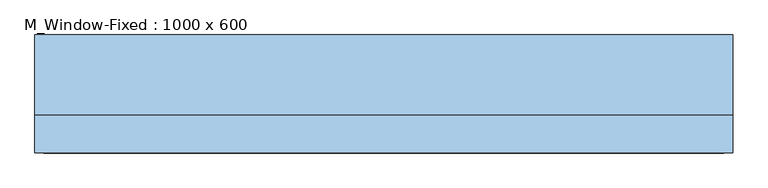
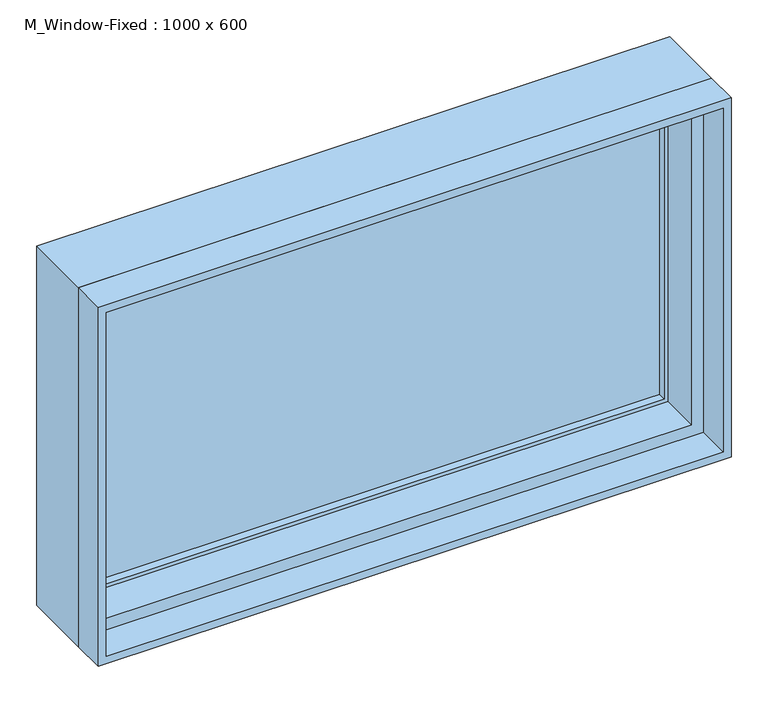
"""IFC4 building model written with IfcOpenShell, lengths in millimetres: window geometry, M_Window-Fixed : 1000 x 600."""

from ifc_helpers import new_model, si_unit, frame, origin, place, context, project, spatial, polyline, outline, extrude, faceted_brep, source, transform, mapped, element, save


def m_window_fixed_1000_x_600_225995cc(model_context):
    return source(origin(), model_context, "Body", "SolidModel", [
        faceted_brep([(500.0, -20.25, 1500.0), (500.0, 94.05, 1500.0), (-500.0, 94.05, 1500.0), (-500.0, -20.25, 1500.0), (-500.0, 94.05, 900.0), (-500.0, -20.25, 900.0), (500.0, 94.05, 900.0), (500.0, -20.25, 900.0), (468.25, -20.25, 1468.25), (468.25, -20.25, 931.75), (-468.25, -20.25, 931.75), (-468.25, -20.25, 1468.25), (-487.3, 94.05, 1487.3), (-487.3, 94.05, 912.7), (487.3, 94.05, 912.7), (487.3, 94.05, 1487.3), (468.25, 43.25, 1468.25), (-468.25, 43.25, 1468.25), (487.3, 43.25, 1487.3), (-487.3, 43.25, 1487.3), (-468.25, 43.25, 931.75), (-487.3, 43.25, 912.7), (468.25, 43.25, 931.75), (487.3, 43.25, 912.7)], [[[0, 1, 2, 3]], [[3, 2, 4, 5]], [[5, 4, 6, 7]], [[3, 5, 7, 0], [8, 9, 10, 11]], [[7, 6, 1, 0]], [[1, 6, 4, 2], [12, 13, 14, 15]], [[16, 8, 11, 17]], [[15, 18, 19, 12]], [[17, 11, 10, 20]], [[12, 19, 21, 13]], [[20, 10, 9, 22]], [[13, 21, 23, 14]], [[22, 9, 8, 16]], [[18, 23, 21, 19], [17, 20, 22, 16]], [[14, 23, 18, 15]]]),
        extrude(outline(polyline([(1500.0, -500.0), (900.0, -500.0), (900.0, 500.0), (1500.0, 500.0), (1500.0, -500.0)]), holes=[polyline([(1487.3, 487.3), (912.7, 487.3), (912.7, -487.3), (1487.3, -487.3), (1487.3, 487.3)])]), frame((0.0, -75.0, 0.0), z_axis=(0.0, 1.0, 0.0), x_axis=(0.0, 0.0, 1.0)), (0.0, 0.0, 1.0), 54.75),
        extrude(outline(polyline([(912.7, 487.3), (1487.3, 487.3), (1487.3, -487.3), (912.7, -487.3), (912.7, 487.3)]), holes=[polyline([(938.1, -461.9), (1461.9, -461.9), (1461.9, 461.9), (938.1, 461.9), (938.1, -461.9)])]), frame((0.0, 43.25, 0.0), z_axis=(0.0, 1.0, 0.0), x_axis=(0.0, 0.0, 1.0)), (0.0, 0.0, 1.0), 44.45),
        extrude(outline(polyline([(461.9, 75.0), (461.9, 68.65), (-461.9, 68.65), (-461.9, 75.0), (461.9, 75.0)])), frame((0.0, 0.0, 938.1), z_axis=(0.0, 0.0, 1.0), x_axis=(1.0, 0.0, 0.0)), (0.0, 0.0, 1.0), 523.8),
        extrude(outline(polyline([(-461.9, 55.95), (-461.9, 62.3), (461.9, 62.3), (461.9, 55.95), (-461.9, 55.95)])), frame((0.0, 0.0, 938.1), z_axis=(0.0, 0.0, 1.0), x_axis=(1.0, 0.0, 0.0)), (0.0, 0.0, 1.0), 523.8),
    ])


if __name__ == "__main__":
    model = new_model("IFC4")
    model_context = context("Model", 3, world=origin())
    ifc_project = project(units=[si_unit("LENGTHUNIT", "METRE", prefix="MILLI")], contexts=[model_context])
    site = spatial("IfcSite", under=ifc_project)
    building = spatial("IfcBuilding", under=site)
    placement = place(None, origin())
    m_window_fixed_1000_x_600_shape = m_window_fixed_1000_x_600_225995cc(model_context)
    element("IfcWindow", 1, ObjectType="M_Window-Fixed : 1000 x 600", at=placement, inside=building, context=model_context, shape_type="MappedRepresentation", body=[
        mapped(m_window_fixed_1000_x_600_shape, transform((0.0, 0.0, 0.0), x_axis=(1.0, 0.0, 0.0), y_axis=(0.0, 1.0, 0.0), z_axis=(0.0, 0.0, 1.0))),
    ])
    save(model, "model.ifc")

# Revit data of these elements
# Type "M_Window-Fixed : 1000 x 600"
#   Type Mark = "42"
#   Fire Rating = "0.5h"
#   Assembly Code = "B2020100"
#   Analytic Construction = "Double glazing - domestic"
#   Window Inset [instance default] = 0 mm
#   Wall Thickness [instance default] = 150 mm
#   Visual Light Transmittance = 0.81
#   Thermal Resistance (R) = 0.319569 (m²·K)/W
#   Solar Heat Gain Coefficient = 0.76
#   Rough Width = 1015 mm
#   Rough Height = 615 mm
#   Interior Wall Closure [instance default] = 54.75 mm
#   Height = 600 mm
#   Heat Transfer Coefficient (U) = 3.12929 W/(m²·K)
#   Frame Extension [instance default] = 6.35 mm
#   Exterior Wall Closure [instance default] = 31.75 mm
#   Extension Jamb [instance default] = 54.75 mm
#   Default Sill Height = 900 mm
#   Width = 1000 mm
#   Muntin Visibility = yes
#   Interior Trim Visibility [instance default] = yes
#   Exterior Trim Visibility [instance default] = yes
#   Extension Jamb Visibility [instance default] = yes
#   Muntin Pattern = M_Muntin Pattern_2x2 : M_Muntin Pattern_2x2
#   Interior Trim Material = Wood - Stained
#   Interior Trim = M_Trim-Window-Interior-Flat : Picture Frame
#   Interior Frame Material = Wood - Stained
#   Glass Panel Material = Glass
#   Exterior Trim Material = Clad - White
#   Exterior Trim = M_Trim-Window-Exterior-Flat : with Sill
#   Exterior Frame Material = Clad - White
#   Wall Closure = (empty or 0)
# Element 1 (IfcWindow, "M_Window-Fixed : 1000 x 600")
#   Materials on its faces: "Wood - Stained", "Glass", "Clad - White"
# Materials
#   "Wood - Stained": class "Wood", colour RGB 173 132 96, transparency 0, Cost = 0
#   "Glass": class "Glass", colour RGB 245 245 243, transparency 1, Description = "Soda Lime Glass", Cost = 0
#   "Clad - White": class "Wood", colour RGB 245 245 243, transparency 0, Cost = 0
